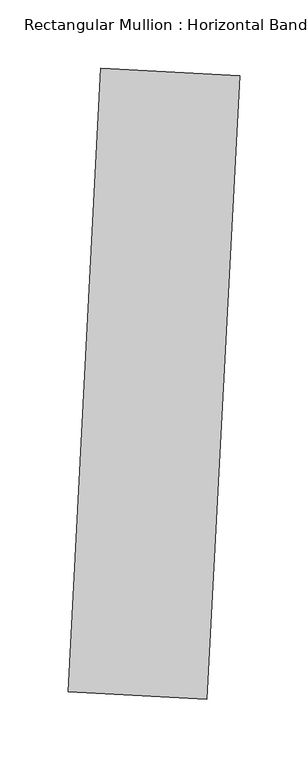
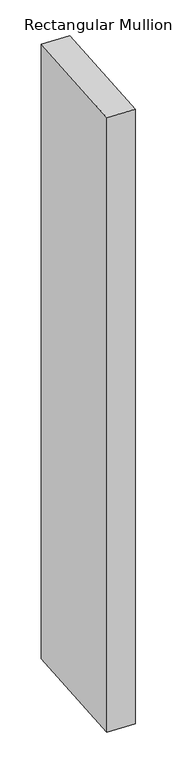
"""IFC4 building model written with IfcOpenShell, lengths in millimetres: member geometry, Rectangular Mullion : Horizontal Band."""

import ifcopenshell
import ifcopenshell.guid

model = None  # the IFC model being written
_history = None  # IfcOwnerHistory: only IFC2X3 demands one
_inside = {}  # id of a spatial element -> (the spatial element, [elements in it])
_under = {}  # id of a project, library or spatial element -> (it, [spatial elements below it])
_declared = {}  # id of a project -> (the project, [libraries it declares])
_typed = {}  # id of a type object -> (the type object, [elements of that type])
_made_of = {}  # id of a material, layer set ... -> (it, [elements and type objects made of it])


def new_model(schema):
    """Start an empty IFC model of exactly this schema.

    Asked for "IFC4X3", IfcOpenShell would pick the latest addendum, in which some entities
    have other attributes; the version numbers below select the first issue.
    IFC2X3 requires an IfcOwnerHistory on every rooted entity: one is made here for all.
    """
    global model, _history
    if schema == "IFC4X3":
        model = ifcopenshell.file(schema_version=(4, 3, 0, 0))
    else:
        model = ifcopenshell.file(schema=schema)
    _inside.clear()
    _under.clear()
    _declared.clear()
    _typed.clear()
    _made_of.clear()
    _history = None
    if model.schema == "IFC2X3":
        org = make("IfcOrganization", Name="unknown")
        user = make(
            "IfcPersonAndOrganization",
            ThePerson=make("IfcPerson", FamilyName="unknown"),
            TheOrganization=org,
        )
        app = make(
            "IfcApplication",
            ApplicationDeveloper=org,
            Version="unknown",
            ApplicationFullName="unknown",
            ApplicationIdentifier="unknown",
        )
        _history = make(
            "IfcOwnerHistory",
            OwningUser=user,
            OwningApplication=app,
            ChangeAction="ADDED",
            CreationDate=0,
        )
    return model


def make(cls, **values):
    """One entity of the class cls with the attributes given. An attribute that is None is left unset."""
    return model.create_entity(
        cls, **{name: value for name, value in values.items() if value is not None}
    )


def rooted(cls, **values):
    """An entity with a GlobalId (a new one), such as an element, a storey or a relation."""
    return make(cls, GlobalId=ifcopenshell.guid.new(), OwnerHistory=_history, **values)


def si_unit(unit_type, name, prefix=None):
    """IfcSIUnit, for example si_unit("LENGTHUNIT", "METRE", prefix="MILLI")."""
    return make("IfcSIUnit", UnitType=unit_type, Prefix=prefix, Name=name)


def assignment(units):
    """IfcUnitAssignment: the units of a project."""
    return None if units is None else make("IfcUnitAssignment", Units=units)


def point(xyz):
    """IfcCartesianPoint."""
    return None if xyz is None else make("IfcCartesianPoint", Coordinates=xyz)


def direction(xyz):
    """IfcDirection."""
    return None if xyz is None else make("IfcDirection", DirectionRatios=xyz)


def frame(location, z_axis=None, x_axis=None):
    """IfcAxis2Placement3D, a coordinate frame: its origin and axes. An axis left out is left unset."""
    return make(
        "IfcAxis2Placement3D",
        Location=point(location),
        Axis=direction(z_axis),
        RefDirection=direction(x_axis),
    )


def origin():
    """The frame at (0, 0, 0) with its axes left unset."""
    return frame((0.0, 0.0, 0.0))


def place(relative_to, where):
    """IfcLocalPlacement: puts the frame where relative to a parent placement (None: the world)."""
    return make(
        "IfcLocalPlacement", PlacementRelTo=relative_to, RelativePlacement=where
    )


def context(
    kind, dimensions, precision=None, world=None, true_north=None, identifier=None
):
    """IfcGeometricRepresentationContext, for example the 3D "Model" context."""
    return make(
        "IfcGeometricRepresentationContext",
        ContextIdentifier=identifier,
        ContextType=kind,
        CoordinateSpaceDimension=dimensions,
        Precision=precision,
        WorldCoordinateSystem=world,
        TrueNorth=true_north,
    )


def project(units=None, contexts=None):
    """IfcProject with its units and contexts."""
    return rooted(
        "IfcProject",
        Name="project",
        RepresentationContexts=contexts,
        UnitsInContext=assignment(units),
    )


def spatial(cls, under=None, at=None, **own):
    """A site, building, storey or space (cls), placed at a placement, below another one or the project."""
    s = rooted(cls, ObjectPlacement=at, **own)
    if under is not None:
        _under.setdefault(under.id(), (under, []))[1].append(s)
    return s


def polyline(points):
    """IfcPolyline through the points."""
    return make("IfcPolyline", Points=[point(p) for p in points])


def outline(outer, holes=None, kind="AREA"):
    """IfcArbitraryClosedProfileDef: a profile drawn as a closed curve; with holes, ...WithVoids."""
    if holes is None:
        return make("IfcArbitraryClosedProfileDef", ProfileType=kind, OuterCurve=outer)
    return make(
        "IfcArbitraryProfileDefWithVoids",
        ProfileType=kind,
        OuterCurve=outer,
        InnerCurves=holes,
    )


def extrude(swept, where, along, depth):
    """IfcExtrudedAreaSolid: the profile swept, set in the frame where, extruded along a direction by depth."""
    return make(
        "IfcExtrudedAreaSolid",
        SweptArea=swept,
        Position=where,
        ExtrudedDirection=direction(along),
        Depth=depth,
    )


def shape(context_of_items, identifier, shape_type, items):
    """IfcShapeRepresentation: the items that make up one representation, for example the "Body"."""
    return make(
        "IfcShapeRepresentation",
        ContextOfItems=context_of_items,
        RepresentationIdentifier=identifier,
        RepresentationType=shape_type,
        Items=items,
    )


def source(mapping_origin, context_of_items, identifier, shape_type, items):
    """IfcRepresentationMap: a shape defined once, which mapped items show again and again."""
    return make(
        "IfcRepresentationMap",
        MappingOrigin=mapping_origin,
        MappedRepresentation=shape(context_of_items, identifier, shape_type, items),
    )


def transform(
    local_origin,
    x_axis=None,
    y_axis=None,
    z_axis=None,
    scale=None,
    scale2=None,
    scale3=None,
    uniform=True,
):
    """IfcCartesianTransformationOperator3D, or its non-uniform kind. x_axis, y_axis, z_axis: its Axis1, 2, 3."""
    if uniform:
        return make(
            "IfcCartesianTransformationOperator3D",
            Axis1=direction(x_axis),
            Axis2=direction(y_axis),
            LocalOrigin=point(local_origin),
            Scale=scale,
            Axis3=direction(z_axis),
        )
    return make(
        "IfcCartesianTransformationOperator3DnonUniform",
        Axis1=direction(x_axis),
        Axis2=direction(y_axis),
        LocalOrigin=point(local_origin),
        Scale=scale,
        Axis3=direction(z_axis),
        Scale2=scale2,
        Scale3=scale3,
    )


def mapped(mapping_source, mapping_target):
    """IfcMappedItem: shows the shape of a source again, moved by a transform."""
    return make(
        "IfcMappedItem", MappingSource=mapping_source, MappingTarget=mapping_target
    )


def made_of(thing, what):
    """Note that an element or type object is made of a material, layer set ...; save() writes the relation."""
    if what is not None:
        _made_of.setdefault(what.id(), (what, []))[1].append(thing)
    return thing


def element(
    cls,
    number,
    at=None,
    inside=None,
    cuts=None,
    type_object=None,
    material=None,
    context=None,
    identifier="Body",
    shape_type=None,
    held_by="IfcProductDefinitionShape",
    body=None,
    shapes=None,
    **own,
):
    """One element of the class cls, such as IfcWall. Its Tag is "e" and its number.

    at: its placement. inside: the storey or other place that contains it. cuts: it is an
    opening in that element (IfcRelVoidsElement). A single representation is given by context,
    identifier, shape_type and body (its items); several are given by shapes. held_by: the class
    of the entity that holds the representations. save() writes the other relations.
    """
    e = rooted(cls, Tag="e%d" % number, ObjectPlacement=at, **own)
    if body is not None:
        shapes = [shape(context, identifier, shape_type, body)]
    if shapes is not None:
        e.Representation = make(held_by, Representations=shapes)
    if inside is not None:
        _inside.setdefault(inside.id(), (inside, []))[1].append(e)
    if cuts is not None:
        rooted(
            "IfcRelVoidsElement", RelatingBuildingElement=cuts, RelatedOpeningElement=e
        )
    if type_object is not None:
        _typed.setdefault(type_object.id(), (type_object, []))[1].append(e)
    return made_of(e, material)


def aggregate(whole, parts):
    """IfcRelAggregates: a whole, such as a stair, and the parts it consists of."""
    return rooted("IfcRelAggregates", RelatingObject=whole, RelatedObjects=parts)


def save(model, path):
    """Write the relations noted so far, then the file.

    IfcRelAggregates (storeys below a building ...), IfcRelContainedInSpatialStructure (elements
    in a storey), IfcRelDefinesByType, IfcRelAssociatesMaterial and IfcRelDeclares: one each for
    every whole, place, type object, material and project.
    """
    for whole, parts in _under.values():
        aggregate(whole, parts)
    for where, things in _inside.values():
        rooted(
            "IfcRelContainedInSpatialStructure",
            RelatedElements=things,
            RelatingStructure=where,
        )
    for kind, things in _typed.values():
        rooted("IfcRelDefinesByType", RelatedObjects=things, RelatingType=kind)
    for what, things in _made_of.values():
        rooted("IfcRelAssociatesMaterial", RelatedObjects=things, RelatingMaterial=what)
    for by, libraries in _declared.values():
        rooted("IfcRelDeclares", RelatingContext=by, RelatedDefinitions=libraries)
    model.write(path)


def rectangular_mullion_horizontal_band_f074a7b8(model_context):
    return source(origin(), model_context, "Body", "SweptSolid", [
        extrude(outline(polyline([(62.69438, 301.8280451), (38.7663808, -154.7453782), (-62.69438, -149.4280451), (-38.7663808, 307.1453782), (62.69438, 301.8280451)])), frame((0.0, 0.0, -2382.029342), z_axis=(0.0, 0.0, 1.0), x_axis=(1.0, 0.0, 0.0)), (0.0, 0.0, 1.0), 2382.029342),
    ])


if __name__ == "__main__":
    model = new_model("IFC4")
    model_context = context("Model", 3, world=origin())
    ifc_project = project(units=[si_unit("LENGTHUNIT", "METRE", prefix="MILLI")], contexts=[model_context])
    site = spatial("IfcSite", under=ifc_project)
    building = spatial("IfcBuilding", under=site)
    placement = place(None, origin())
    rectangular_mullion_horizontal_band_shape = rectangular_mullion_horizontal_band_f074a7b8(model_context)
    element("IfcMember", 1, ObjectType="Rectangular Mullion : Horizontal Band", at=placement, inside=building, context=model_context, shape_type="MappedRepresentation", body=[
        mapped(rectangular_mullion_horizontal_band_shape, transform((0.0, 0.0, 0.0), x_axis=(1.0, 0.0, 0.0), y_axis=(0.0, 1.0, 0.0), z_axis=(0.0, 0.0, 1.0))),
    ])
    save(model, "model.ifc")

# Revit data of these elements
# Type "Rectangular Mullion : Horizontal Band"
#   built-in parameter 1007351 = 0.25 (stored number, unit not read)
#   built-in parameter 1007304 = 1.5 (stored number, unit not read)
#   built-in parameter 1007301 = 0.166667 (stored number, unit not read)
#   built-in parameter 1007300 = 0.166667 (stored number, unit not read)
# Element 1 (IfcMember, "Rectangular Mullion : Horizontal Band")
#   Materials on its faces: "Aluminum"
# Materials
#   "Aluminum": class "Metal", colour RGB 247 247 247, transparency 0, Description = "Aluminum 6061", Cost = 0
